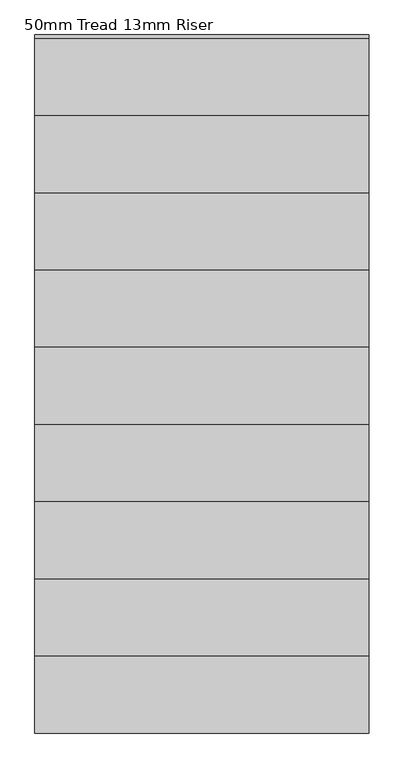
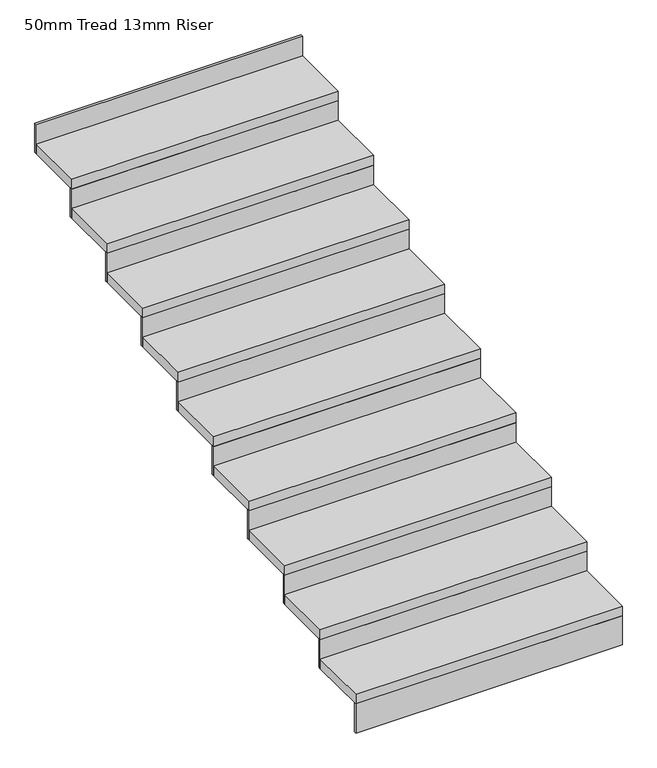
"""IFC4 building model written with IfcOpenShell, lengths in millimetres: stair flight geometry, 50mm Tread 13mm Riser."""

from ifc_helpers import new_model, si_unit, frame, origin, place, context, project, spatial, polyline, outline, extrude, source, transform, mapped, element, save


def stair_flight_50mm_tread_13mm_riser_c35dab0d(model_context):
    return source(origin(), model_context, "Body", "SweptSolid", [
        extrude(outline(polyline([(-13276.101437, -1987.6378151), (-13276.101437, -2000.1378151), (-14576.101437, -2000.1378151), (-14576.101437, -1987.6378151), (-13276.101437, -1987.6378151)])), frame((0.0, 0.0, 1450.0), z_axis=(0.0, 0.0, 1.0), x_axis=(1.0, 0.0, 0.0)), (0.0, 0.0, 1.0), 150.0),
        extrude(outline(polyline([(-14576.101437, -1700.1378151), (-13276.101437, -1700.1378151), (-13276.101437, -2000.1378151), (-14576.101437, -2000.1378151), (-14576.101437, -1700.1378151)])), frame((0.0, 0.0, 1600.0), z_axis=(0.0, 0.0, 1.0), x_axis=(1.0, 0.0, 0.0)), (0.0, 0.0, 1.0), 50.0),
        extrude(outline(polyline([(-13276.101437, -1687.6378151), (-13276.101437, -1700.1378151), (-14576.101437, -1700.1378151), (-14576.101437, -1687.6378151), (-13276.101437, -1687.6378151)])), frame((0.0, 0.0, 1600.0), z_axis=(0.0, 0.0, 1.0), x_axis=(1.0, 0.0, 0.0)), (0.0, 0.0, 1.0), 150.0),
        extrude(outline(polyline([(-14576.101437, -1400.1378151), (-13276.101437, -1400.1378151), (-13276.101437, -1700.1378151), (-14576.101437, -1700.1378151), (-14576.101437, -1400.1378151)])), frame((0.0, 0.0, 1750.0), z_axis=(0.0, 0.0, 1.0), x_axis=(1.0, 0.0, 0.0)), (0.0, 0.0, 1.0), 50.0),
        extrude(outline(polyline([(-13276.101437, -1387.6378151), (-13276.101437, -1400.1378151), (-14576.101437, -1400.1378151), (-14576.101437, -1387.6378151), (-13276.101437, -1387.6378151)])), frame((0.0, 0.0, 1750.0), z_axis=(0.0, 0.0, 1.0), x_axis=(1.0, 0.0, 0.0)), (0.0, 0.0, 1.0), 150.0),
        extrude(outline(polyline([(-14576.101437, -1100.1378151), (-13276.101437, -1100.1378151), (-13276.101437, -1400.1378151), (-14576.101437, -1400.1378151), (-14576.101437, -1100.1378151)])), frame((0.0, 0.0, 1900.0), z_axis=(0.0, 0.0, 1.0), x_axis=(1.0, 0.0, 0.0)), (0.0, 0.0, 1.0), 50.0),
        extrude(outline(polyline([(-13276.101437, -1087.6378151), (-13276.101437, -1100.1378151), (-14576.101437, -1100.1378151), (-14576.101437, -1087.6378151), (-13276.101437, -1087.6378151)])), frame((0.0, 0.0, 1900.0), z_axis=(0.0, 0.0, 1.0), x_axis=(1.0, 0.0, 0.0)), (0.0, 0.0, 1.0), 150.0),
        extrude(outline(polyline([(-14576.101437, -800.1378151), (-13276.101437, -800.1378151), (-13276.101437, -1100.1378151), (-14576.101437, -1100.1378151), (-14576.101437, -800.1378151)])), frame((0.0, 0.0, 2050.0), z_axis=(0.0, 0.0, 1.0), x_axis=(1.0, 0.0, 0.0)), (0.0, 0.0, 1.0), 50.0),
        extrude(outline(polyline([(-13276.101437, -787.6378151), (-13276.101437, -800.1378151), (-14576.101437, -800.1378151), (-14576.101437, -787.6378151), (-13276.101437, -787.6378151)])), frame((0.0, 0.0, 2050.0), z_axis=(0.0, 0.0, 1.0), x_axis=(1.0, 0.0, 0.0)), (0.0, 0.0, 1.0), 150.0),
        extrude(outline(polyline([(-14576.101437, -500.1378151), (-13276.101437, -500.1378151), (-13276.101437, -800.1378151), (-14576.101437, -800.1378151), (-14576.101437, -500.1378151)])), frame((0.0, 0.0, 2200.0), z_axis=(0.0, 0.0, 1.0), x_axis=(1.0, 0.0, 0.0)), (0.0, 0.0, 1.0), 50.0),
        extrude(outline(polyline([(-13276.101437, -487.6378151), (-13276.101437, -500.1378151), (-14576.101437, -500.1378151), (-14576.101437, -487.6378151), (-13276.101437, -487.6378151)])), frame((0.0, 0.0, 2200.0), z_axis=(0.0, 0.0, 1.0), x_axis=(1.0, 0.0, 0.0)), (0.0, 0.0, 1.0), 150.0),
        extrude(outline(polyline([(-14576.101437, -200.1378151), (-13276.101437, -200.1378151), (-13276.101437, -500.1378151), (-14576.101437, -500.1378151), (-14576.101437, -200.1378151)])), frame((0.0, 0.0, 2350.0), z_axis=(0.0, 0.0, 1.0), x_axis=(1.0, 0.0, 0.0)), (0.0, 0.0, 1.0), 50.0),
        extrude(outline(polyline([(-13276.101437, -187.6378151), (-13276.101437, -200.1378151), (-14576.101437, -200.1378151), (-14576.101437, -187.6378151), (-13276.101437, -187.6378151)])), frame((0.0, 0.0, 2350.0), z_axis=(0.0, 0.0, 1.0), x_axis=(1.0, 0.0, 0.0)), (0.0, 0.0, 1.0), 150.0),
        extrude(outline(polyline([(-14576.101437, 99.8621849), (-13276.101437, 99.8621849), (-13276.101437, -200.1378151), (-14576.101437, -200.1378151), (-14576.101437, 99.8621849)])), frame((0.0, 0.0, 2500.0), z_axis=(0.0, 0.0, 1.0), x_axis=(1.0, 0.0, 0.0)), (0.0, 0.0, 1.0), 50.0),
        extrude(outline(polyline([(-13276.101437, 112.3621849), (-13276.101437, 99.8621849), (-14576.101437, 99.8621849), (-14576.101437, 112.3621849), (-13276.101437, 112.3621849)])), frame((0.0, 0.0, 2500.0), z_axis=(0.0, 0.0, 1.0), x_axis=(1.0, 0.0, 0.0)), (0.0, 0.0, 1.0), 150.0),
        extrude(outline(polyline([(-14576.101437, 399.8621849), (-13276.101437, 399.8621849), (-13276.101437, 99.8621849), (-14576.101437, 99.8621849), (-14576.101437, 399.8621849)])), frame((0.0, 0.0, 2650.0), z_axis=(0.0, 0.0, 1.0), x_axis=(1.0, 0.0, 0.0)), (0.0, 0.0, 1.0), 50.0),
        extrude(outline(polyline([(-13276.101437, 412.3621849), (-13276.101437, 399.8621849), (-14576.101437, 399.8621849), (-14576.101437, 412.3621849), (-13276.101437, 412.3621849)])), frame((0.0, 0.0, 2650.0), z_axis=(0.0, 0.0, 1.0), x_axis=(1.0, 0.0, 0.0)), (0.0, 0.0, 1.0), 150.0),
        extrude(outline(polyline([(-13276.101437, 712.3621849), (-13276.101437, 699.8621849), (-14576.101437, 699.8621849), (-14576.101437, 712.3621849), (-13276.101437, 712.3621849)])), frame((0.0, 0.0, 2800.0), z_axis=(0.0, 0.0, 1.0), x_axis=(1.0, 0.0, 0.0)), (0.0, 0.0, 1.0), 150.0),
        extrude(outline(polyline([(-14576.101437, 699.8621849), (-13276.101437, 699.8621849), (-13276.101437, 399.8621849), (-14576.101437, 399.8621849), (-14576.101437, 699.8621849)])), frame((0.0, 0.0, 2800.0), z_axis=(0.0, 0.0, 1.0), x_axis=(1.0, 0.0, 0.0)), (0.0, 0.0, 1.0), 50.0),
    ])


if __name__ == "__main__":
    model = new_model("IFC4")
    model_context = context("Model", 3, world=origin())
    ifc_project = project(units=[si_unit("LENGTHUNIT", "METRE", prefix="MILLI")], contexts=[model_context])
    site = spatial("IfcSite", under=ifc_project)
    building = spatial("IfcBuilding", under=site)
    placement = place(None, origin())
    stair_flight_50mm_tread_13mm_riser_shape = stair_flight_50mm_tread_13mm_riser_c35dab0d(model_context)
    element("IfcStairFlight", 1, ObjectType="50mm Tread 13mm Riser", at=placement, inside=building, context=model_context, shape_type="MappedRepresentation", body=[
        mapped(stair_flight_50mm_tread_13mm_riser_shape, transform((0.0, 0.0, 0.0), x_axis=(1.0, 0.0, 0.0), y_axis=(0.0, 1.0, 0.0), z_axis=(0.0, 0.0, 1.0))),
    ])
    save(model, "model.ifc")
